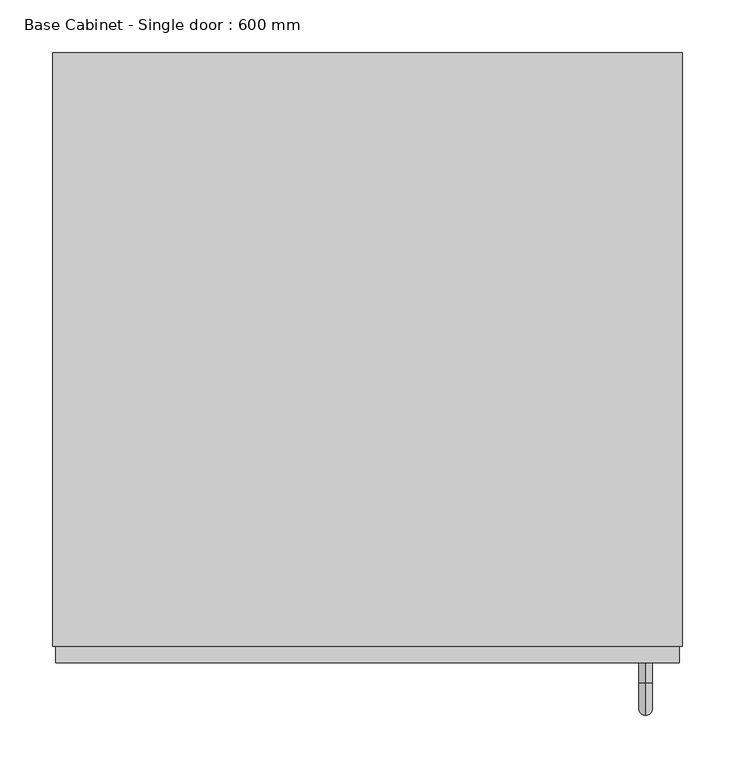
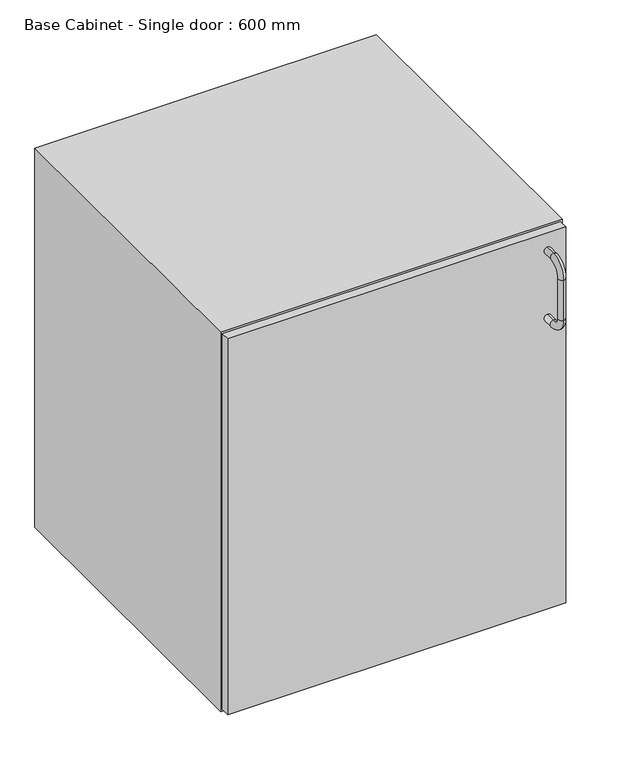
"""IFC4 building model written with IfcOpenShell, lengths in millimetres: furniture geometry, Base Cabinet - Single door : 600 mm."""

from ifc_helpers import new_model, si_unit, point, frame, origin, place, context, project, spatial, polyline, circle_curve, ellipse_curve, trimmed, outline, extrude, source, transform, mapped, element, save
from ifc_brep_helpers import plane_surface, cylinder_surface, revolved_surface, advanced_brep


def base_cabinet_single_door_600_mm_e367a429(model_context):
    return source(origin(), model_context, "Body", "SolidModel", [
        extrude(outline(polyline([(341.7003264, -581.0), (-252.2996736, -581.0), (-252.2996736, -565.0), (341.7003264, -565.0), (341.7003264, -581.0)])), frame((0.0, 0.0, 167.0), z_axis=(0.0, 0.0, 1.0), x_axis=(1.0, 0.0, 0.0)), (0.0, 0.0, 1.0), 698.0),
        advanced_brep(
        [(309.7003264, -581.0, 839.25), (309.7003264, -581.0, 826.75), (309.7003264, -599.75, 839.25), (309.7003264, -599.75, 826.75), (309.7003264, -618.5, 808.0), (309.7003264, -631.0, 808.0), (309.7003264, -631.0, 733.0), (309.7003264, -618.5, 733.0), (309.7003264, -599.75, 714.25), (309.7003264, -599.75, 701.75), (309.7003264, -581.0, 701.75), (309.7003264, -581.0, 714.25)],
        [
            (0, 1, circle_curve(frame((309.7003264, -581.0, 833.0), z_axis=(0.0, 1.0, 0.0), x_axis=(0.0, 0.0, -1.0)), 6.25)),
            (1, 0, circle_curve(frame((309.7003264, -581.0, 833.0), z_axis=(0.0, 1.0, 0.0), x_axis=(0.0, 0.0, -1.0)), 6.25)),
            (0, 2),
            (2, 3, circle_curve(frame((309.7003264, -599.75, 833.0), z_axis=(0.0, 1.0, 0.0), x_axis=(0.0, 0.0, -1.0)), 6.25)),
            (3, 1),
            (3, 2, circle_curve(frame((309.7003264, -599.75, 833.0), z_axis=(0.0, 1.0, 0.0), x_axis=(0.0, 0.0, -1.0)), 6.25)),
            (4, 3, circle_curve(frame((309.7003264, -599.75, 808.0), z_axis=(-1.0, 0.0, 0.0), x_axis=(0.0, 0.0, 1.0)), 18.75)),
            (2, 5, circle_curve(frame((309.7003264, -599.75, 808.0), z_axis=(1.0, 0.0, 0.0), x_axis=(0.0, 0.0, 1.0)), 31.25)),
            (5, 4, circle_curve(frame((309.7003264, -624.75, 808.0), z_axis=(0.0, 0.0, 1.0), x_axis=(0.0, 1.0, 0.0)), 6.25)),
            (4, 5, circle_curve(frame((309.7003264, -624.75, 808.0), z_axis=(0.0, 0.0, 1.0), x_axis=(0.0, 1.0, 0.0)), 6.25)),
            (5, 6),
            (6, 7, circle_curve(frame((309.7003264, -624.75, 733.0), z_axis=(0.0, 0.0, 1.0), x_axis=(0.0, 1.0, 0.0)), 6.25)),
            (7, 4),
            (7, 6, circle_curve(frame((309.7003264, -624.75, 733.0), z_axis=(0.0, 0.0, 1.0), x_axis=(0.0, 1.0, 0.0)), 6.25)),
            (8, 7, circle_curve(frame((309.7003264, -599.75, 733.0), z_axis=(-1.0, 0.0, 0.0), x_axis=(0.0, -1.0, 0.0)), 18.75)),
            (6, 9, circle_curve(frame((309.7003264, -599.75, 733.0), z_axis=(1.0, 0.0, 0.0), x_axis=(0.0, -1.0, 0.0)), 31.25)),
            (9, 8, circle_curve(frame((309.7003264, -599.75, 708.0), z_axis=(0.0, -1.0, 0.0), x_axis=(0.0, 0.0, 1.0)), 6.25)),
            (8, 9, circle_curve(frame((309.7003264, -599.75, 708.0), z_axis=(0.0, -1.0, 0.0), x_axis=(0.0, 0.0, 1.0)), 6.25)),
            (10, 11, circle_curve(frame((309.7003264, -581.0, 708.0), z_axis=(0.0, 1.0, 0.0), x_axis=(0.0, 0.0, 1.0)), 6.25)),
            (11, 10, circle_curve(frame((309.7003264, -581.0, 708.0), z_axis=(0.0, 1.0, 0.0), x_axis=(0.0, 0.0, 1.0)), 6.25)),
            (9, 10),
            (11, 8),
        ],
        [
            plane_surface(frame((309.7003264, -581.0, 833.0), z_axis=(0.0, 1.0, 0.0), x_axis=(1.0, 0.0, 0.0))),
            cylinder_surface(frame((309.7003264, -581.0, 833.0), z_axis=(0.0, 1.0, 0.0), x_axis=(0.0, 0.0, -1.0)), 6.25),
            revolved_surface(trimmed(ellipse_curve(frame((309.7003264, -599.75, 833.0), z_axis=(0.0, 1.0, 0.0), x_axis=(0.0, 0.0, -1.0)), 6.25, 6.25), [point((309.7003264, -599.75, 839.25))], [point((309.7003264, -599.75, 826.75))], True, "CARTESIAN"), (309.7003264, -599.75, 808.0), (1.0, 0.0, 0.0)),
            revolved_surface(trimmed(ellipse_curve(frame((309.7003264, -599.75, 833.0), z_axis=(0.0, 1.0, 0.0), x_axis=(0.0, 0.0, -1.0)), 6.25, 6.25), [point((309.7003264, -599.75, 826.75))], [point((309.7003264, -599.75, 839.25))], True, "CARTESIAN"), (309.7003264, -599.75, 808.0), (1.0, 0.0, 0.0)),
            cylinder_surface(frame((309.7003264, -624.75, 808.0), z_axis=(0.0, 0.0, 1.0), x_axis=(0.0, 1.0, 0.0)), 6.25),
            revolved_surface(trimmed(ellipse_curve(frame((309.7003264, -624.75, 733.0), z_axis=(0.0, 0.0, 1.0), x_axis=(0.0, 1.0, 0.0)), 6.25, 6.25), [point((309.7003264, -631.0, 733.0))], [point((309.7003264, -618.5, 733.0))], True, "CARTESIAN"), (309.7003264, -599.75, 733.0), (1.0, 0.0, 0.0)),
            revolved_surface(trimmed(ellipse_curve(frame((309.7003264, -624.75, 733.0), z_axis=(0.0, 0.0, 1.0), x_axis=(0.0, 1.0, 0.0)), 6.25, 6.25), [point((309.7003264, -618.5, 733.0))], [point((309.7003264, -631.0, 733.0))], True, "CARTESIAN"), (309.7003264, -599.75, 733.0), (1.0, 0.0, 0.0)),
            plane_surface(frame((309.7003264, -581.0, 708.0), z_axis=(0.0, 1.0, 0.0), x_axis=(1.0, 0.0, 0.0))),
            cylinder_surface(frame((309.7003264, -599.75, 708.0), z_axis=(0.0, -1.0, 0.0), x_axis=(0.0, 0.0, 1.0)), 6.25),
        ],
        [
            (0, [[1, 2]]),
            (1, [[-1, 3, 4, 5]]),
            (1, [[-2, -5, 6, -3]]),
            (2, [[7, -4, 8, 9]]),
            (3, [[-8, -6, -7, 10]]),
            (4, [[-9, 11, 12, 13]]),
            (4, [[-10, -13, 14, -11]]),
            (5, [[15, -12, 16, 17]]),
            (6, [[-16, -14, -15, 18]]),
            (7, [[19, 20]]),
            (8, [[-17, 21, -20, 22]]),
            (8, [[-18, -22, -19, -21]]),
        ],
    ),
        extrude(outline(polyline([(868.0, 344.7003264), (868.0, -255.2996736), (164.0, -255.2996736), (164.0, 344.7003264), (868.0, 344.7003264)]), holes=[polyline([(852.0, 328.7003264), (180.0, 328.7003264), (180.0, -239.2996736), (852.0, -239.2996736), (852.0, 328.7003264)])]), frame((0.0, -565.0, 0.0), z_axis=(0.0, 1.0, 0.0), x_axis=(0.0, 0.0, 1.0)), (0.0, 0.0, 1.0), 565.0),
        extrude(outline(polyline([(328.7003264, -16.0), (-239.2996736, -16.0), (-239.2996736, -10.0), (328.7003264, -10.0), (328.7003264, -16.0)])), frame((0.0, 0.0, 180.0), z_axis=(0.0, 0.0, 1.0), x_axis=(1.0, 0.0, 0.0)), (0.0, 0.0, 1.0), 672.0),
    ])


if __name__ == "__main__":
    model = new_model("IFC4")
    model_context = context("Model", 3, world=origin())
    ifc_project = project(units=[si_unit("LENGTHUNIT", "METRE", prefix="MILLI")], contexts=[model_context])
    site = spatial("IfcSite", under=ifc_project)
    building = spatial("IfcBuilding", under=site)
    placement = place(None, origin())
    base_cabinet_single_door_600_mm_shape = base_cabinet_single_door_600_mm_e367a429(model_context)
    element("IfcFurniture", 1, ObjectType="Base Cabinet - Single door : 600 mm", at=placement, inside=building, context=model_context, shape_type="MappedRepresentation", body=[
        mapped(base_cabinet_single_door_600_mm_shape, transform((0.0, 0.0, 0.0), x_axis=(1.0, 0.0, 0.0), y_axis=(0.0, 1.0, 0.0), z_axis=(0.0, 0.0, 1.0))),
    ])
    save(model, "model.ifc")

# Revit data of these elements
# Type "Base Cabinet - Single door : 600 mm"
#   Creator Organization [instance default] = "© Danish Educational Content"
#   Creator Name [instance default] = "© Erik Falck Jørgensen"
#   Creator Build [instance default] = "2023.0405.0"
#   Width = 600 mm
#   Sink Cut Hole [instance default] = 5 mm
#   Sink Cut Distance [instance default] = 130 mm
#   Plinth Height = 164 mm
#   Height = 704 mm
#   Handle From Top = 35 mm
#   Handle From Side = 35 mm
#   Handle Angle = 90.00°
#   Front Thickness = 16 mm
#   Cabinet Thickness = 16 mm
#   Depth = 565 mm
#   Swing = yes
#   Sink Cut [instance default] = no
#   Masking = yes
#   Casework = yes
#   Handle Finish = none
#   Handle [instance default] = element 685946
#   Front Finish = none
#   Front [instance default] = element 685947
#   Cabinet Finish = none
#   Default Elevation = 0
#   Assembly Code = ""
# Element 1 (IfcFurniture, "Base Cabinet - Single door : 600 mm")
#   Materials on its faces: "Default Casework (Interior)", "Stainless Steel, Polished"
# Materials
#   "Default Casework (Interior)": class "Generic", colour RGB 205 205 205, transparency 0, Description = "Udefineret element materiale", Cost = 0
#   "Stainless Steel, Polished": class "Metal", colour RGB 180 180 180, transparency 0, Description = "Rustfri stål, poleret", Cost = 0
